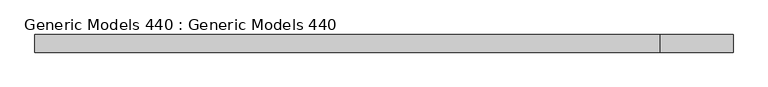
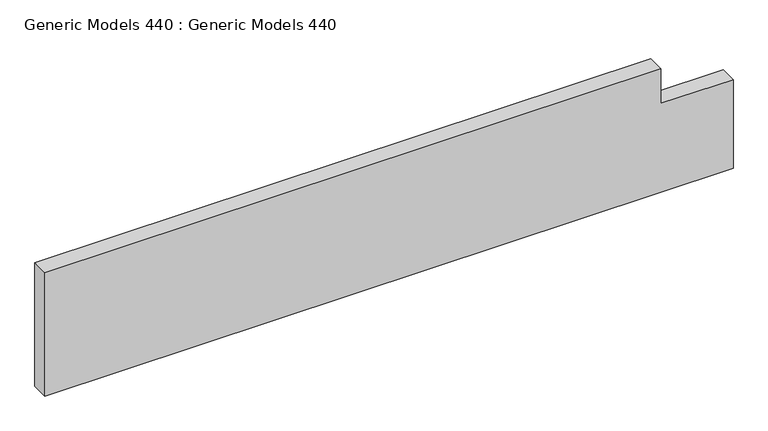
"""IFC4 building model written with IfcOpenShell, lengths in millimetres: proxy geometry, Generic Models 440 : Generic Models 440."""

from ifc_helpers import new_model, si_unit, frame, origin, place, context, project, spatial, polyline, outline, extrude, source, transform, mapped, element, save


def generic_models_440_generic_models_440_a3a74885(model_context):
    return source(origin(), model_context, "Body", "SweptSolid", [
        extrude(outline(polyline([(126377.446, -8128.1736296), (126377.446, -6619.9216296), (126582.9668961, -6619.9216296), (126582.9668961, -6778.6716296), (126663.196, -6778.6716296), (126663.196, -8128.1736296), (126377.446, -8128.1736296)])), frame((0.0, 542.3477803, 0.0), z_axis=(0.0, 1.0, 0.0), x_axis=(0.0, 0.0, 1.0)), (0.0, 0.0, 1.0), 38.1),
    ])


if __name__ == "__main__":
    model = new_model("IFC4")
    model_context = context("Model", 3, world=origin())
    ifc_project = project(units=[si_unit("LENGTHUNIT", "METRE", prefix="MILLI")], contexts=[model_context])
    site = spatial("IfcSite", under=ifc_project)
    building = spatial("IfcBuilding", under=site)
    placement = place(None, origin())
    generic_models_440_generic_models_440_shape = generic_models_440_generic_models_440_a3a74885(model_context)
    element("IfcBuildingElementProxy", 1, Name="Generic Models 440 : Generic Models 440", ObjectType="Generic Models 440 : Generic Models 440", at=placement, inside=building, context=model_context, shape_type="MappedRepresentation", body=[
        mapped(generic_models_440_generic_models_440_shape, transform((0.0, 0.0, 0.0), x_axis=(1.0, 0.0, 0.0), y_axis=(0.0, 1.0, 0.0), z_axis=(0.0, 0.0, 1.0))),
    ])
    save(model, "model.ifc")

# Revit data of these elements
# Element 1 (IfcBuildingElementProxy, "Generic Models 440 : Generic Models 440")
#   Materials on its faces: "_STRUCTURAL MEMBER (SEE STRUCT. DWGS)"
# Materials
#   "_STRUCTURAL MEMBER (SEE STRUCT. DWGS)": class "Generic", colour RGB 209 182 141, transparency 0, Cost = 0
